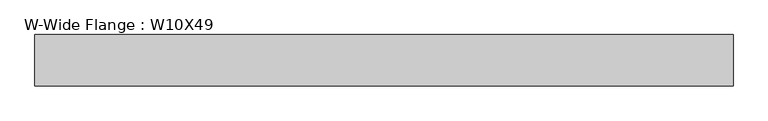
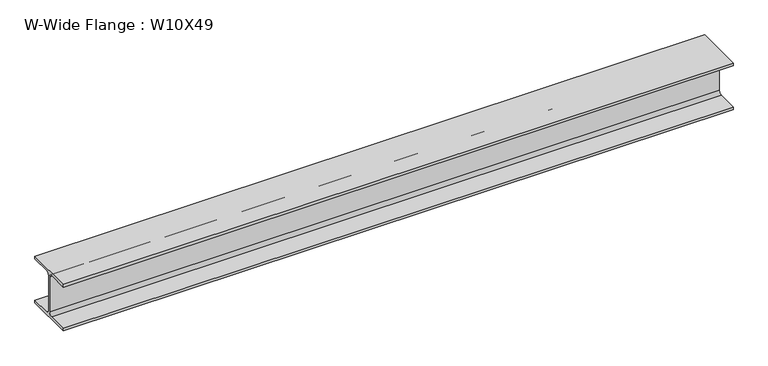
"""IFC4 building model written with IfcOpenShell, lengths in millimetres: beam geometry, W-Wide Flange : W10X49."""

from ifc_helpers import new_model, si_unit, point, frame, frame_2d, origin, place, context, project, spatial, polyline, circle_curve, trimmed, segment, composite_curve, outline, extrude, source, transform, mapped, element, save


def w_wide_flange_w10x49_01df90bb(model_context):
    return source(origin(), model_context, "Body", "SweptSolid", [
        extrude(outline(composite_curve([segment(polyline([(127.0, -112.776), (127.0, -127.0), (-127.0, -127.0), (-127.0, -112.776), (-21.844, -112.776)]), True, "CONTINUOUS"), segment(trimmed(circle_curve(frame_2d((-21.844, -95.25)), 17.526), [point((-21.844, -112.776))], [point((-4.318, -95.25))], True, "CARTESIAN"), True, "CONTINUOUS"), segment(polyline([(-4.318, -95.25), (-4.318, 95.25)]), True, "CONTINUOUS"), segment(trimmed(circle_curve(frame_2d((-21.844, 95.25)), 17.526), [point((-4.318, 95.25))], [point((-21.844, 112.776))], True, "CARTESIAN"), True, "CONTINUOUS"), segment(polyline([(-21.844, 112.776), (-127.0, 112.776), (-127.0, 127.0), (127.0, 127.0), (127.0, 112.776), (21.844, 112.776)]), True, "CONTINUOUS"), segment(trimmed(circle_curve(frame_2d((21.844, 95.25)), 17.526), [point((21.844, 112.776))], [point((4.318, 95.25))], True, "CARTESIAN"), True, "CONTINUOUS"), segment(polyline([(4.318, 95.25), (4.318, -95.25)]), True, "CONTINUOUS"), segment(trimmed(circle_curve(frame_2d((21.844, -95.25)), 17.526), [point((4.318, -95.25))], [point((21.844, -112.776))], True, "CARTESIAN"), True, "CONTINUOUS"), segment(polyline([(21.844, -112.776), (127.0, -112.776)]), True, "CONTINUOUS")], self_intersect=False)), frame((-1754.1378906, 0.0, 0.0), z_axis=(1.0, 0.0, 0.0), x_axis=(0.0, 1.0, 0.0)), (0.0, 0.0, 1.0), 3458.2695313),
    ])


if __name__ == "__main__":
    model = new_model("IFC4")
    model_context = context("Model", 3, world=origin())
    ifc_project = project(units=[si_unit("LENGTHUNIT", "METRE", prefix="MILLI")], contexts=[model_context])
    site = spatial("IfcSite", under=ifc_project)
    building = spatial("IfcBuilding", under=site)
    placement = place(None, origin())
    w_wide_flange_w10x49_shape = w_wide_flange_w10x49_01df90bb(model_context)
    element("IfcBeam", 1, ObjectType="W-Wide Flange : W10X49", at=placement, inside=building, context=model_context, shape_type="MappedRepresentation", body=[
        mapped(w_wide_flange_w10x49_shape, transform((0.0, 0.0, 0.0), x_axis=(1.0, 0.0, 0.0), y_axis=(0.0, 1.0, 0.0), z_axis=(0.0, 0.0, 1.0))),
    ])
    save(model, "model.ifc")

# Revit data of these elements
# Type "W-Wide Flange : W10X49"
#   Assembly Code = "B10"
#   W = 49
#   Length [instance default] = 1524 mm
#   bf = 254 mm
#   d = 254 mm
#   k = 31.75 mm
#   k2 = 17.526 mm
#   tf = 14.224 mm
#   tw = 8.636 mm
#   A = 0.0092903 m²
#   Structural Material [instance default] = Steel ASTM A992
# Element 1 (IfcBeam, "W-Wide Flange : W10X49")
#   Structural Material = Aluminum, Anodized Red
#   Materials on its faces: "Aluminum, Anodized Red"
# Materials
#   "Steel ASTM A992": class "Metal", colour RGB 128 0 0, transparency 0, Description = "Structural steel 50ksi", Cost = 0
#   "Aluminum, Anodized Red": class "Metal", colour RGB 120 120 120, transparency 0, Description = "Anodized aluminum, red", Cost = 0
